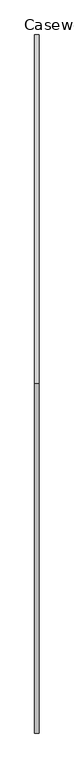
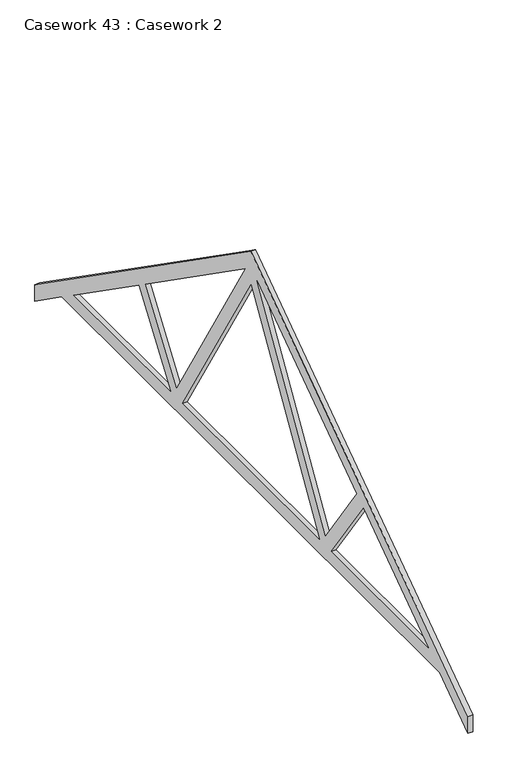
"""IFC4 building model written with IfcOpenShell, lengths in millimetres: furniture geometry, Casework 43 : Casework 2."""

import ifcopenshell
import ifcopenshell.guid

model = None  # the IFC model being written
_history = None  # IfcOwnerHistory: only IFC2X3 demands one
_inside = {}  # id of a spatial element -> (the spatial element, [elements in it])
_under = {}  # id of a project, library or spatial element -> (it, [spatial elements below it])
_declared = {}  # id of a project -> (the project, [libraries it declares])
_typed = {}  # id of a type object -> (the type object, [elements of that type])
_made_of = {}  # id of a material, layer set ... -> (it, [elements and type objects made of it])


def new_model(schema):
    """Start an empty IFC model of exactly this schema.

    Asked for "IFC4X3", IfcOpenShell would pick the latest addendum, in which some entities
    have other attributes; the version numbers below select the first issue.
    IFC2X3 requires an IfcOwnerHistory on every rooted entity: one is made here for all.
    """
    global model, _history
    if schema == "IFC4X3":
        model = ifcopenshell.file(schema_version=(4, 3, 0, 0))
    else:
        model = ifcopenshell.file(schema=schema)
    _inside.clear()
    _under.clear()
    _declared.clear()
    _typed.clear()
    _made_of.clear()
    _history = None
    if model.schema == "IFC2X3":
        org = make("IfcOrganization", Name="unknown")
        user = make(
            "IfcPersonAndOrganization",
            ThePerson=make("IfcPerson", FamilyName="unknown"),
            TheOrganization=org,
        )
        app = make(
            "IfcApplication",
            ApplicationDeveloper=org,
            Version="unknown",
            ApplicationFullName="unknown",
            ApplicationIdentifier="unknown",
        )
        _history = make(
            "IfcOwnerHistory",
            OwningUser=user,
            OwningApplication=app,
            ChangeAction="ADDED",
            CreationDate=0,
        )
    return model


def make(cls, **values):
    """One entity of the class cls with the attributes given. An attribute that is None is left unset."""
    return model.create_entity(
        cls, **{name: value for name, value in values.items() if value is not None}
    )


def rooted(cls, **values):
    """An entity with a GlobalId (a new one), such as an element, a storey or a relation."""
    return make(cls, GlobalId=ifcopenshell.guid.new(), OwnerHistory=_history, **values)


def si_unit(unit_type, name, prefix=None):
    """IfcSIUnit, for example si_unit("LENGTHUNIT", "METRE", prefix="MILLI")."""
    return make("IfcSIUnit", UnitType=unit_type, Prefix=prefix, Name=name)


def assignment(units):
    """IfcUnitAssignment: the units of a project."""
    return None if units is None else make("IfcUnitAssignment", Units=units)


def point(xyz):
    """IfcCartesianPoint."""
    return None if xyz is None else make("IfcCartesianPoint", Coordinates=xyz)


def direction(xyz):
    """IfcDirection."""
    return None if xyz is None else make("IfcDirection", DirectionRatios=xyz)


def frame(location, z_axis=None, x_axis=None):
    """IfcAxis2Placement3D, a coordinate frame: its origin and axes. An axis left out is left unset."""
    return make(
        "IfcAxis2Placement3D",
        Location=point(location),
        Axis=direction(z_axis),
        RefDirection=direction(x_axis),
    )


def origin():
    """The frame at (0, 0, 0) with its axes left unset."""
    return frame((0.0, 0.0, 0.0))


def place(relative_to, where):
    """IfcLocalPlacement: puts the frame where relative to a parent placement (None: the world)."""
    return make(
        "IfcLocalPlacement", PlacementRelTo=relative_to, RelativePlacement=where
    )


def context(
    kind, dimensions, precision=None, world=None, true_north=None, identifier=None
):
    """IfcGeometricRepresentationContext, for example the 3D "Model" context."""
    return make(
        "IfcGeometricRepresentationContext",
        ContextIdentifier=identifier,
        ContextType=kind,
        CoordinateSpaceDimension=dimensions,
        Precision=precision,
        WorldCoordinateSystem=world,
        TrueNorth=true_north,
    )


def project(units=None, contexts=None):
    """IfcProject with its units and contexts."""
    return rooted(
        "IfcProject",
        Name="project",
        RepresentationContexts=contexts,
        UnitsInContext=assignment(units),
    )


def spatial(cls, under=None, at=None, **own):
    """A site, building, storey or space (cls), placed at a placement, below another one or the project."""
    s = rooted(cls, ObjectPlacement=at, **own)
    if under is not None:
        _under.setdefault(under.id(), (under, []))[1].append(s)
    return s


def polyline(points):
    """IfcPolyline through the points."""
    return make("IfcPolyline", Points=[point(p) for p in points])


def outline(outer, holes=None, kind="AREA"):
    """IfcArbitraryClosedProfileDef: a profile drawn as a closed curve; with holes, ...WithVoids."""
    if holes is None:
        return make("IfcArbitraryClosedProfileDef", ProfileType=kind, OuterCurve=outer)
    return make(
        "IfcArbitraryProfileDefWithVoids",
        ProfileType=kind,
        OuterCurve=outer,
        InnerCurves=holes,
    )


def extrude(swept, where, along, depth):
    """IfcExtrudedAreaSolid: the profile swept, set in the frame where, extruded along a direction by depth."""
    return make(
        "IfcExtrudedAreaSolid",
        SweptArea=swept,
        Position=where,
        ExtrudedDirection=direction(along),
        Depth=depth,
    )


def shape(context_of_items, identifier, shape_type, items):
    """IfcShapeRepresentation: the items that make up one representation, for example the "Body"."""
    return make(
        "IfcShapeRepresentation",
        ContextOfItems=context_of_items,
        RepresentationIdentifier=identifier,
        RepresentationType=shape_type,
        Items=items,
    )


def source(mapping_origin, context_of_items, identifier, shape_type, items):
    """IfcRepresentationMap: a shape defined once, which mapped items show again and again."""
    return make(
        "IfcRepresentationMap",
        MappingOrigin=mapping_origin,
        MappedRepresentation=shape(context_of_items, identifier, shape_type, items),
    )


def transform(
    local_origin,
    x_axis=None,
    y_axis=None,
    z_axis=None,
    scale=None,
    scale2=None,
    scale3=None,
    uniform=True,
):
    """IfcCartesianTransformationOperator3D, or its non-uniform kind. x_axis, y_axis, z_axis: its Axis1, 2, 3."""
    if uniform:
        return make(
            "IfcCartesianTransformationOperator3D",
            Axis1=direction(x_axis),
            Axis2=direction(y_axis),
            LocalOrigin=point(local_origin),
            Scale=scale,
            Axis3=direction(z_axis),
        )
    return make(
        "IfcCartesianTransformationOperator3DnonUniform",
        Axis1=direction(x_axis),
        Axis2=direction(y_axis),
        LocalOrigin=point(local_origin),
        Scale=scale,
        Axis3=direction(z_axis),
        Scale2=scale2,
        Scale3=scale3,
    )


def mapped(mapping_source, mapping_target):
    """IfcMappedItem: shows the shape of a source again, moved by a transform."""
    return make(
        "IfcMappedItem", MappingSource=mapping_source, MappingTarget=mapping_target
    )


def made_of(thing, what):
    """Note that an element or type object is made of a material, layer set ...; save() writes the relation."""
    if what is not None:
        _made_of.setdefault(what.id(), (what, []))[1].append(thing)
    return thing


def element(
    cls,
    number,
    at=None,
    inside=None,
    cuts=None,
    type_object=None,
    material=None,
    context=None,
    identifier="Body",
    shape_type=None,
    held_by="IfcProductDefinitionShape",
    body=None,
    shapes=None,
    **own,
):
    """One element of the class cls, such as IfcWall. Its Tag is "e" and its number.

    at: its placement. inside: the storey or other place that contains it. cuts: it is an
    opening in that element (IfcRelVoidsElement). A single representation is given by context,
    identifier, shape_type and body (its items); several are given by shapes. held_by: the class
    of the entity that holds the representations. save() writes the other relations.
    """
    e = rooted(cls, Tag="e%d" % number, ObjectPlacement=at, **own)
    if body is not None:
        shapes = [shape(context, identifier, shape_type, body)]
    if shapes is not None:
        e.Representation = make(held_by, Representations=shapes)
    if inside is not None:
        _inside.setdefault(inside.id(), (inside, []))[1].append(e)
    if cuts is not None:
        rooted(
            "IfcRelVoidsElement", RelatingBuildingElement=cuts, RelatedOpeningElement=e
        )
    if type_object is not None:
        _typed.setdefault(type_object.id(), (type_object, []))[1].append(e)
    return made_of(e, material)


def aggregate(whole, parts):
    """IfcRelAggregates: a whole, such as a stair, and the parts it consists of."""
    return rooted("IfcRelAggregates", RelatingObject=whole, RelatedObjects=parts)


def save(model, path):
    """Write the relations noted so far, then the file.

    IfcRelAggregates (storeys below a building ...), IfcRelContainedInSpatialStructure (elements
    in a storey), IfcRelDefinesByType, IfcRelAssociatesMaterial and IfcRelDeclares: one each for
    every whole, place, type object, material and project.
    """
    for whole, parts in _under.values():
        aggregate(whole, parts)
    for where, things in _inside.values():
        rooted(
            "IfcRelContainedInSpatialStructure",
            RelatedElements=things,
            RelatingStructure=where,
        )
    for kind, things in _typed.values():
        rooted("IfcRelDefinesByType", RelatedObjects=things, RelatingType=kind)
    for what, things in _made_of.values():
        rooted("IfcRelAssociatesMaterial", RelatedObjects=things, RelatingMaterial=what)
    for by, libraries in _declared.values():
        rooted("IfcRelDeclares", RelatingContext=by, RelatedDefinitions=libraries)
    model.write(path)


def casework_43_casework_2_e74e5d3e(model_context):
    return source(origin(), model_context, "Body", "SweptSolid", [
        extrude(outline(polyline([(6583.1149316, 5257.5), (-277.3850684, 5257.5), (-786.6126654, 4900.9349979), (-786.6126654, 5084.0511862), (3152.8649316, 7842.5030963), (7073.1149316, 5097.5144946), (7073.1149316, 4914.3983063), (6583.1149316, 5257.5)]), holes=[polyline([(4612.3149663, 5407.5), (6368.8927306, 5407.5), (5190.2113591, 6232.8215815), (4612.3149663, 5407.5)]), polyline([(4394.2037684, 5407.5), (3152.8649316, 7473.4347567), (1911.5260948, 5407.5), (4394.2037684, 5407.5)]), polyline([(4504.5438357, 5515.1038939), (5067.3385525, 6318.8580469), (3262.0771677, 7582.915677), (4504.5438357, 5515.1038939)]), polyline([(1693.4148969, 5407.5), (1115.5185041, 6232.8215815), (-63.1628674, 5407.5), (1693.4148969, 5407.5)]), polyline([(1801.1860276, 5515.1038939), (3043.6526956, 7582.915677), (1238.3913108, 6318.8580469), (1801.1860276, 5515.1038939)])]), frame((-8621.5247381, 0.0, 0.0), z_axis=(1.0, 0.0, 0.0), x_axis=(0.0, 1.0, 0.0)), (0.0, 0.0, 1.0), 49.6351915),
    ])


if __name__ == "__main__":
    model = new_model("IFC4")
    model_context = context("Model", 3, world=origin())
    ifc_project = project(units=[si_unit("LENGTHUNIT", "METRE", prefix="MILLI")], contexts=[model_context])
    site = spatial("IfcSite", under=ifc_project)
    building = spatial("IfcBuilding", under=site)
    placement = place(None, origin())
    casework_43_casework_2_shape = casework_43_casework_2_e74e5d3e(model_context)
    element("IfcFurniture", 1, ObjectType="Casework 43 : Casework 2", at=placement, inside=building, context=model_context, shape_type="MappedRepresentation", body=[
        mapped(casework_43_casework_2_shape, transform((0.0, 0.0, 0.0), x_axis=(1.0, 0.0, 0.0), y_axis=(0.0, 1.0, 0.0), z_axis=(0.0, 0.0, 1.0))),
    ])
    save(model, "model.ifc")

# Revit data of these elements
# Element 1 (IfcFurniture, "Casework 43 : Casework 2")
#   Materials on its faces: "Softwood, Lumber"
# Materials
#   "Softwood, Lumber": class "Wood", colour RGB 205 156 65, transparency 0, Description = "Pinus Echinata", Cost = 0
